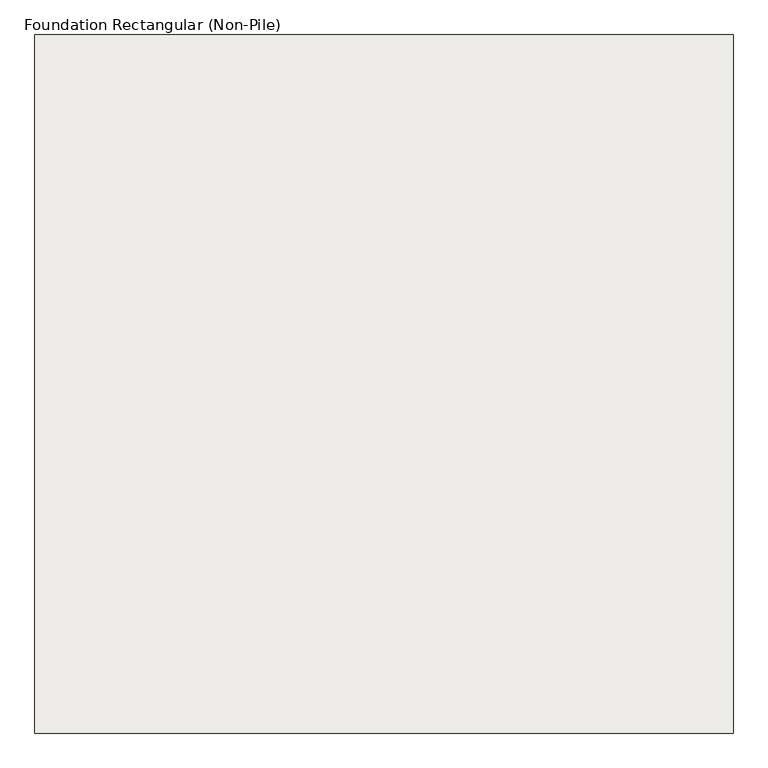
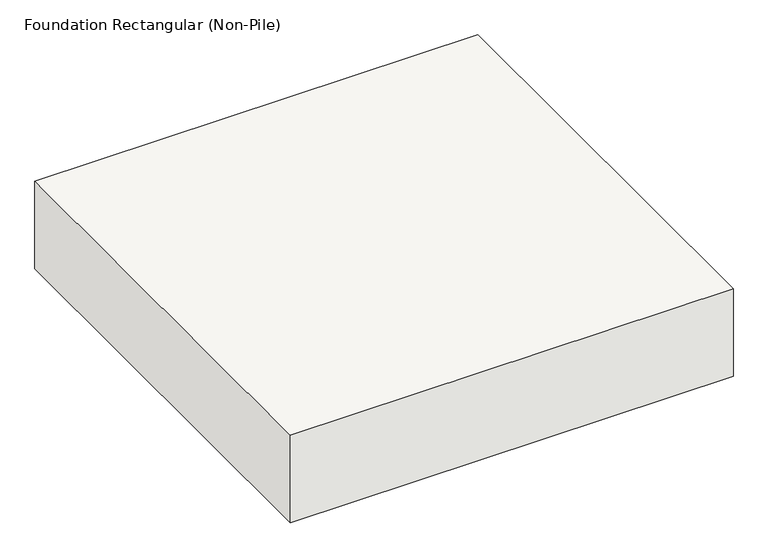
"""IFC4 building model written with IfcOpenShell, lengths in millimetres: slab geometry, Foundation Rectangular (Non-Pile) : H_SF_AR_S18_W2400xL2400xT500_Bitumen."""

from ifc_helpers import new_model, si_unit, frame, origin, place, context, project, spatial, polyline, outline, extrude, source, transform, mapped, element, save


def foundation_rectangular_non_pile_5fe39465(model_context):
    return source(origin(), model_context, "Body", "SweptSolid", [
        extrude(outline(polyline([(1200.0, 1200.0), (1200.0, -1200.0), (-1200.0, -1200.0), (-1200.0, 1200.0), (1200.0, 1200.0)])), frame((0.0, 0.0, -500.0), z_axis=(0.0, 0.0, 1.0), x_axis=(1.0, 0.0, 0.0)), (0.0, 0.0, 1.0), 500.0),
    ])


if __name__ == "__main__":
    model = new_model("IFC4")
    model_context = context("Model", 3, world=origin())
    ifc_project = project(units=[si_unit("LENGTHUNIT", "METRE", prefix="MILLI")], contexts=[model_context])
    site = spatial("IfcSite", under=ifc_project)
    building = spatial("IfcBuilding", under=site)
    placement = place(None, origin())
    foundation_rectangular_non_pile_shape = foundation_rectangular_non_pile_5fe39465(model_context)
    element("IfcSlab", 1, ObjectType="Foundation Rectangular (Non-Pile) : H_SF_AR_S18_W2400xL2400xT500_Bitumen", at=placement, inside=building, context=model_context, shape_type="MappedRepresentation", body=[
        mapped(foundation_rectangular_non_pile_shape, transform((0.0, 0.0, 0.0), x_axis=(1.0, 0.0, 0.0), y_axis=(0.0, 1.0, 0.0), z_axis=(0.0, 0.0, 1.0))),
    ])
    save(model, "model.ifc")

# Revit data of these elements
# Type "Foundation Rectangular (Non-Pile) : H_SF_AR_S18_W2400xL2400xT500_Bitumen"
#   Top bar = "D25@300"
#   Description = "UG Shallow Foundation"
#   Bottom bar = "D20@300"
#   Width = 2400 mm
#   Length = 2400 mm
#   Foundation Thickness = 500 mm
#   Structural Material [instance default] = none
#   Assembly Code = ""
